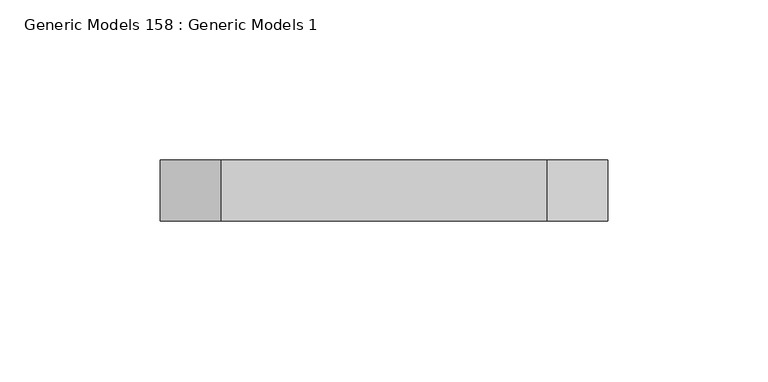
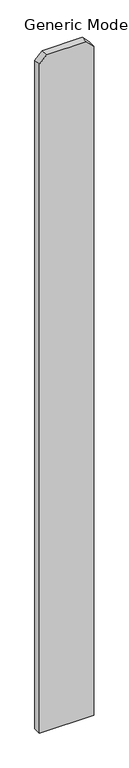
"""IFC4 building model written with IfcOpenShell, lengths in millimetres: proxy geometry, Generic Models 158 : Generic Models 1."""

from ifc_helpers import new_model, si_unit, frame, origin, place, context, project, spatial, polyline, outline, extrude, source, transform, mapped, element, save


def generic_models_158_generic_models_1_ac1548d8(model_context):
    return source(origin(), model_context, "Body", "SweptSolid", [
        extrude(outline(polyline([(76.2, -250724.9875), (1885.95, -250724.9875), (1905.0, -250744.0375), (1905.0, -250845.6375), (1885.95, -250864.6875), (76.2, -250864.6875), (76.2, -250724.9875)])), frame((0.0, 547.6875, 0.0), z_axis=(0.0, 1.0, 0.0), x_axis=(0.0, 0.0, 1.0)), (0.0, 0.0, 1.0), 19.05),
    ])


if __name__ == "__main__":
    model = new_model("IFC4")
    model_context = context("Model", 3, world=origin())
    ifc_project = project(units=[si_unit("LENGTHUNIT", "METRE", prefix="MILLI")], contexts=[model_context])
    site = spatial("IfcSite", under=ifc_project)
    building = spatial("IfcBuilding", under=site)
    placement = place(None, origin())
    generic_models_158_generic_models_1_shape = generic_models_158_generic_models_1_ac1548d8(model_context)
    element("IfcBuildingElementProxy", 1, Name="Generic Models 158 : Generic Models 1", ObjectType="Generic Models 158 : Generic Models 1", at=placement, inside=building, context=model_context, shape_type="MappedRepresentation", body=[
        mapped(generic_models_158_generic_models_1_shape, transform((0.0, 0.0, 0.0), x_axis=(1.0, 0.0, 0.0), y_axis=(0.0, 1.0, 0.0), z_axis=(0.0, 0.0, 1.0))),
    ])
    save(model, "model.ifc")

# Revit data of these elements
# Element 1 (IfcBuildingElementProxy, "Generic Models 158 : Generic Models 1")
#   Materials on its faces: "VERTICAL 1X6 CEDAR PLANKS W/ CLEAR WOOD SEALER"
# Materials
#   "VERTICAL 1X6 CEDAR PLANKS W/ CLEAR WOOD SEALER": class "Wood", colour RGB 234 198 147, transparency 0, Description = "Pinus Echinata", Cost = 0
